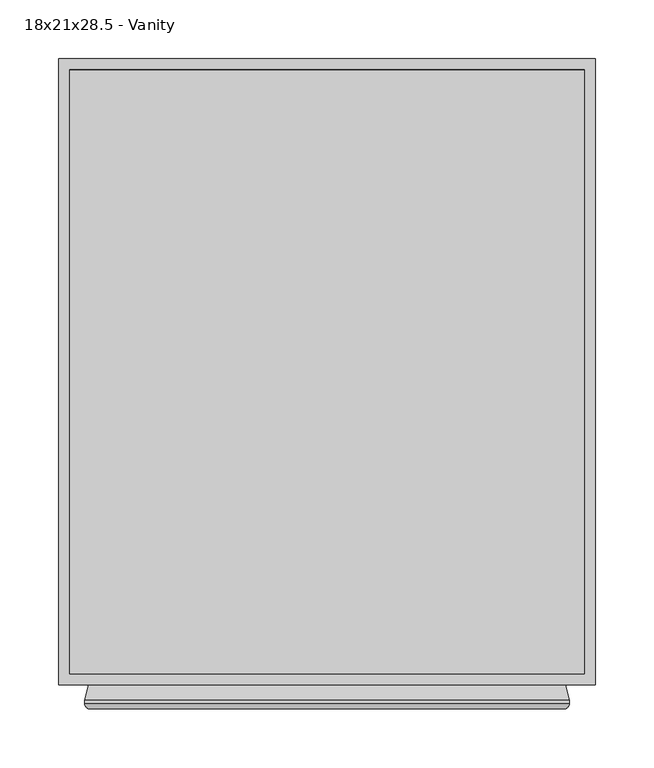
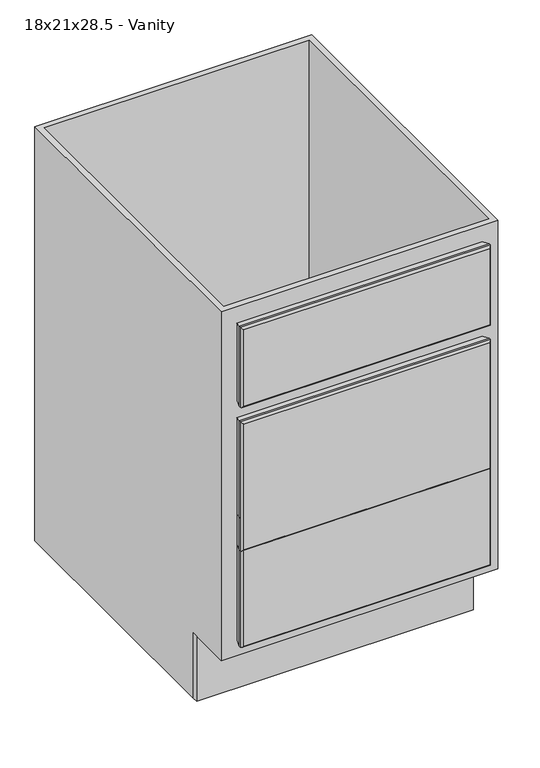
"""IFC4 building model written with IfcOpenShell, lengths in millimetres: furniture geometry, Cabinet-Base-Merillat-Three_Drawer-Marlin : 18x21x28.5 - Vanity."""

from ifc_helpers import new_model, si_unit, frame, origin, origin_with_axes, place, context, project, spatial, polyline, ellipse_curve, outline, extrude, faceted_brep, source, transform, mapped, element, save
from ifc_brep_helpers import plane_surface, cylinder_surface, advanced_brep


def furniture_18x21x28_5_vanity_0f894329(model_context):
    return source(origin(), model_context, "Body", "SolidModel", [
        advanced_brep(
        [(-184.5408026, -629.92, 530.3035075), (-184.5408026, -629.92, 311.0714925), (222.0162124, -629.92, 311.0714925), (222.0162124, -629.92, 530.3035075), (-184.1320951, -609.6, 311.4802), (-184.1320951, -609.6, 529.8948), (221.6075049, -609.6, 529.8948), (221.6075049, -609.6, 311.4802), (-187.6372951, -625.4496, 533.4), (-187.6372951, -622.681, 533.4), (-187.6372951, -622.681, 307.975), (-187.6372951, -625.4496, 307.975), (225.1127049, -622.681, 307.975), (225.1127049, -625.4496, 307.975), (225.1127049, -622.681, 533.4), (225.1127049, -625.4496, 533.4)],
        [
            (0, 1),
            (1, 2),
            (2, 3),
            (3, 0),
            (4, 5),
            (5, 6),
            (6, 7),
            (7, 4),
            (8, 9),
            (9, 10),
            (10, 11),
            (11, 8),
            (10, 12),
            (12, 13),
            (13, 11),
            (12, 14),
            (14, 15),
            (15, 13),
            (8, 15),
            (14, 9),
            (11, 1, ellipse_curve(frame((-182.8620951, -625.4496, 312.7502), z_axis=(-0.7071067811865475, 0.0, 0.7071067811865475), x_axis=(-0.7071067811865474, 0.0, -0.7071067811865476)), 6.7531526, 4.7752)),
            (0, 8, ellipse_curve(frame((-182.8620951, -625.4496, 528.6248), z_axis=(-0.7071067811865475, 0.0, -0.7071067811865475), x_axis=(0.7071067811865474, 0.0, -0.7071067811865476)), 6.7531526, 4.7752)),
            (4, 10),
            (9, 5),
            (13, 2, ellipse_curve(frame((220.3375049, -625.4496, 312.7502), z_axis=(-0.7071067811865475, 0.0, -0.7071067811865475), x_axis=(0.7071067811865476, 0.0, -0.7071067811865474)), 6.7531526, 4.7752)),
            (7, 12),
            (15, 3, ellipse_curve(frame((220.3375049, -625.4496, 528.6248), z_axis=(0.7071067811865475, 0.0, -0.7071067811865475), x_axis=(0.7071067811865474, 0.0, 0.7071067811865476)), 6.7531526, 4.7752)),
            (6, 14),
        ],
        [
            plane_surface(frame((-187.6372951, -629.92, 533.4), z_axis=(0.0, -1.0, 0.0), x_axis=(0.0, 0.0, -1.0))),
            plane_surface(frame((-187.6372951, -609.6, 533.4), z_axis=(0.0, 1.0, 0.0), x_axis=(0.0, 0.0, 1.0))),
            plane_surface(frame((-187.6372951, -629.92, 533.4), z_axis=(-1.0, 0.0, 0.0), x_axis=(0.0, 1.0, 0.0))),
            plane_surface(frame((-187.6372951, -629.92, 307.975), z_axis=(0.0, 0.0, -1.0), x_axis=(0.0, 1.0, 0.0))),
            plane_surface(frame((225.1127049, -629.92, 307.975), z_axis=(1.0, 0.0, 0.0), x_axis=(0.0, 1.0, 0.0))),
            plane_surface(frame((225.1127049, -629.92, 533.4), z_axis=(0.0, 0.0, 1.0), x_axis=(0.0, 1.0, 0.0))),
            cylinder_surface(frame((-182.8620951, -625.4496, 533.4), z_axis=(0.0, 0.0, -1.0), x_axis=(0.0, 1.0, 0.0)), 4.7752),
            plane_surface(frame((-187.6372951, -622.681, 533.4), z_axis=(-0.9659229350723619, 0.25882983502910506, 0.0), x_axis=(0.0, 0.0, -1.0))),
            cylinder_surface(frame((-187.6372951, -625.4496, 312.7502), z_axis=(1.0, 0.0, 0.0), x_axis=(0.0, 1.0, 0.0)), 4.7752),
            plane_surface(frame((-187.6372951, -622.681, 307.975), z_axis=(0.0, 0.25882983502910506, -0.9659229350723619), x_axis=(1.0, 0.0, 0.0))),
            cylinder_surface(frame((220.3375049, -625.4496, 307.975), z_axis=(0.0, 0.0, 1.0), x_axis=(0.0, 1.0, 0.0)), 4.7752),
            plane_surface(frame((225.1127049, -622.681, 307.975), z_axis=(0.9659229350723619, 0.25882983502910506, 0.0), x_axis=(0.0, 0.0, 1.0))),
            cylinder_surface(frame((225.1127049, -625.4496, 528.6248), z_axis=(-1.0, 0.0, 0.0), x_axis=(0.0, 1.0, 0.0)), 4.7752),
            plane_surface(frame((225.1127049, -622.681, 533.4), z_axis=(0.0, 0.25882983502910506, 0.9659229350723619), x_axis=(-1.0, 0.0, 0.0))),
        ],
        [
            (0, [[1, 2, 3, 4]]),
            (1, [[5, 6, 7, 8]]),
            (2, [[9, 10, 11, 12]]),
            (3, [[-11, 13, 14, 15]]),
            (4, [[-14, 16, 17, 18]]),
            (5, [[-9, 19, -17, 20]]),
            (6, [[21, -1, 22, -12]]),
            (7, [[23, -10, 24, -5]]),
            (8, [[-21, -15, 25, -2]]),
            (9, [[-23, -8, 26, -13]]),
            (10, [[-25, -18, 27, -3]]),
            (11, [[-26, -7, 28, -16]]),
            (12, [[-22, -4, -27, -19]]),
            (13, [[-24, -20, -28, -6]]),
        ],
    ),
        advanced_brep(
        [(-184.5408026, -629.92, 695.4035075), (-184.5408026, -629.92, 561.8964925), (222.0162124, -629.92, 561.8964925), (222.0162124, -629.92, 695.4035075), (-184.1320951, -609.6, 562.3052), (-184.1320951, -609.6, 694.9948), (221.6075049, -609.6, 694.9948), (221.6075049, -609.6, 562.3052), (-187.6372951, -625.4496, 698.5), (-187.6372951, -622.681, 698.5), (-187.6372951, -622.681, 558.8), (-187.6372951, -625.4496, 558.8), (225.1127049, -622.681, 558.8), (225.1127049, -625.4496, 558.8), (225.1127049, -622.681, 698.5), (225.1127049, -625.4496, 698.5)],
        [
            (0, 1),
            (1, 2),
            (2, 3),
            (3, 0),
            (4, 5),
            (5, 6),
            (6, 7),
            (7, 4),
            (8, 9),
            (9, 10),
            (10, 11),
            (11, 8),
            (10, 12),
            (12, 13),
            (13, 11),
            (12, 14),
            (14, 15),
            (15, 13),
            (8, 15),
            (14, 9),
            (11, 1, ellipse_curve(frame((-182.8620951, -625.4496, 563.5752), z_axis=(-0.7071067811865475, 0.0, 0.7071067811865475), x_axis=(-0.7071067811865474, 0.0, -0.7071067811865476)), 6.7531526, 4.7752)),
            (0, 8, ellipse_curve(frame((-182.8620951, -625.4496, 693.7248), z_axis=(-0.7071067811865475, 0.0, -0.7071067811865475), x_axis=(0.7071067811865474, 0.0, -0.7071067811865476)), 6.7531526, 4.7752)),
            (4, 10),
            (9, 5),
            (13, 2, ellipse_curve(frame((220.3375049, -625.4496, 563.5752), z_axis=(-0.7071067811865475, 0.0, -0.7071067811865475), x_axis=(0.7071067811865476, 0.0, -0.7071067811865474)), 6.7531526, 4.7752)),
            (7, 12),
            (15, 3, ellipse_curve(frame((220.3375049, -625.4496, 693.7248), z_axis=(0.7071067811865475, 0.0, -0.7071067811865475), x_axis=(0.7071067811865474, 0.0, 0.7071067811865476)), 6.7531526, 4.7752)),
            (6, 14),
        ],
        [
            plane_surface(frame((-187.6372951, -629.92, 698.5), z_axis=(0.0, -1.0, 0.0), x_axis=(0.0, 0.0, -1.0))),
            plane_surface(frame((-187.6372951, -609.6, 698.5), z_axis=(0.0, 1.0, 0.0), x_axis=(0.0, 0.0, 1.0))),
            plane_surface(frame((-187.6372951, -629.92, 698.5), z_axis=(-1.0, 0.0, 0.0), x_axis=(0.0, 1.0, 0.0))),
            plane_surface(frame((-187.6372951, -629.92, 558.8), z_axis=(0.0, 0.0, -1.0), x_axis=(0.0, 1.0, 0.0))),
            plane_surface(frame((225.1127049, -629.92, 558.8), z_axis=(1.0, 0.0, 0.0), x_axis=(0.0, 1.0, 0.0))),
            plane_surface(frame((225.1127049, -629.92, 698.5), z_axis=(0.0, 0.0, 1.0), x_axis=(0.0, 1.0, 0.0))),
            cylinder_surface(frame((-182.8620951, -625.4496, 698.5), z_axis=(0.0, 0.0, -1.0), x_axis=(0.0, 1.0, 0.0)), 4.7752),
            plane_surface(frame((-187.6372951, -622.681, 698.5), z_axis=(-0.9659229350723619, 0.25882983502910506, 0.0), x_axis=(0.0, 0.0, -1.0))),
            cylinder_surface(frame((-187.6372951, -625.4496, 563.5752), z_axis=(1.0, 0.0, 0.0), x_axis=(0.0, 1.0, 0.0)), 4.7752),
            plane_surface(frame((-187.6372951, -622.681, 558.8), z_axis=(0.0, 0.25882983502910506, -0.9659229350723619), x_axis=(1.0, 0.0, 0.0))),
            cylinder_surface(frame((220.3375049, -625.4496, 558.8), z_axis=(0.0, 0.0, 1.0), x_axis=(0.0, 1.0, 0.0)), 4.7752),
            plane_surface(frame((225.1127049, -622.681, 558.8), z_axis=(0.9659229350723619, 0.25882983502910506, 0.0), x_axis=(0.0, 0.0, 1.0))),
            cylinder_surface(frame((225.1127049, -625.4496, 693.7248), z_axis=(-1.0, 0.0, 0.0), x_axis=(0.0, 1.0, 0.0)), 4.7752),
            plane_surface(frame((225.1127049, -622.681, 698.5), z_axis=(0.0, 0.25882983502910506, 0.9659229350723619), x_axis=(-1.0, 0.0, 0.0))),
        ],
        [
            (0, [[1, 2, 3, 4]]),
            (1, [[5, 6, 7, 8]]),
            (2, [[9, 10, 11, 12]]),
            (3, [[-11, 13, 14, 15]]),
            (4, [[-14, 16, 17, 18]]),
            (5, [[-9, 19, -17, 20]]),
            (6, [[21, -1, 22, -12]]),
            (7, [[23, -10, 24, -5]]),
            (8, [[-21, -15, 25, -2]]),
            (9, [[-23, -8, 26, -13]]),
            (10, [[-25, -18, 27, -3]]),
            (11, [[-26, -7, 28, -16]]),
            (12, [[-22, -4, -27, -19]]),
            (13, [[-24, -20, -28, -6]]),
        ],
    ),
        advanced_brep(
        [(-184.5408026, -629.92, 362.0285075), (-184.5408026, -629.92, 142.7964925), (222.0162124, -629.92, 142.7964925), (222.0162124, -629.92, 362.0285075), (-184.1320951, -609.6, 143.2052), (-184.1320951, -609.6, 361.6198), (221.6075049, -609.6, 361.6198), (221.6075049, -609.6, 143.2052), (-187.6372951, -625.4496, 365.125), (-187.6372951, -622.681, 365.125), (-187.6372951, -622.681, 139.7), (-187.6372951, -625.4496, 139.7), (225.1127049, -622.681, 139.7), (225.1127049, -625.4496, 139.7), (225.1127049, -622.681, 365.125), (225.1127049, -625.4496, 365.125)],
        [
            (0, 1),
            (1, 2),
            (2, 3),
            (3, 0),
            (4, 5),
            (5, 6),
            (6, 7),
            (7, 4),
            (8, 9),
            (9, 10),
            (10, 11),
            (11, 8),
            (10, 12),
            (12, 13),
            (13, 11),
            (12, 14),
            (14, 15),
            (15, 13),
            (8, 15),
            (14, 9),
            (11, 1, ellipse_curve(frame((-182.8620951, -625.4496, 144.4752), z_axis=(-0.7071067811865475, 0.0, 0.7071067811865475), x_axis=(-0.7071067811865474, 0.0, -0.7071067811865476)), 6.7531526, 4.7752)),
            (0, 8, ellipse_curve(frame((-182.8620951, -625.4496, 360.3498), z_axis=(-0.7071067811865475, 0.0, -0.7071067811865475), x_axis=(0.7071067811865474, 0.0, -0.7071067811865476)), 6.7531526, 4.7752)),
            (4, 10),
            (9, 5),
            (13, 2, ellipse_curve(frame((220.3375049, -625.4496, 144.4752), z_axis=(-0.7071067811865475, 0.0, -0.7071067811865475), x_axis=(0.7071067811865476, 0.0, -0.7071067811865474)), 6.7531526, 4.7752)),
            (7, 12),
            (15, 3, ellipse_curve(frame((220.3375049, -625.4496, 360.3498), z_axis=(0.7071067811865475, 0.0, -0.7071067811865475), x_axis=(0.7071067811865474, 0.0, 0.7071067811865476)), 6.7531526, 4.7752)),
            (6, 14),
        ],
        [
            plane_surface(frame((-187.6372951, -629.92, 365.125), z_axis=(0.0, -1.0, 0.0), x_axis=(0.0, 0.0, -1.0))),
            plane_surface(frame((-187.6372951, -609.6, 365.125), z_axis=(0.0, 1.0, 0.0), x_axis=(0.0, 0.0, 1.0))),
            plane_surface(frame((-187.6372951, -629.92, 365.125), z_axis=(-1.0, 0.0, 0.0), x_axis=(0.0, 1.0, 0.0))),
            plane_surface(frame((-187.6372951, -629.92, 139.7), z_axis=(0.0, 0.0, -1.0), x_axis=(0.0, 1.0, 0.0))),
            plane_surface(frame((225.1127049, -629.92, 139.7), z_axis=(1.0, 0.0, 0.0), x_axis=(0.0, 1.0, 0.0))),
            plane_surface(frame((225.1127049, -629.92, 365.125), z_axis=(0.0, 0.0, 1.0), x_axis=(0.0, 1.0, 0.0))),
            cylinder_surface(frame((-182.8620951, -625.4496, 365.125), z_axis=(0.0, 0.0, -1.0), x_axis=(0.0, 1.0, 0.0)), 4.7752),
            plane_surface(frame((-187.6372951, -622.681, 365.125), z_axis=(-0.9659229350723619, 0.25882983502910506, 0.0), x_axis=(0.0, 0.0, -1.0))),
            cylinder_surface(frame((-187.6372951, -625.4496, 144.4752), z_axis=(1.0, 0.0, 0.0), x_axis=(0.0, 1.0, 0.0)), 4.7752),
            plane_surface(frame((-187.6372951, -622.681, 139.7), z_axis=(0.0, 0.25882983502910506, -0.9659229350723619), x_axis=(1.0, 0.0, 0.0))),
            cylinder_surface(frame((220.3375049, -625.4496, 139.7), z_axis=(0.0, 0.0, 1.0), x_axis=(0.0, 1.0, 0.0)), 4.7752),
            plane_surface(frame((225.1127049, -622.681, 139.7), z_axis=(0.9659229350723619, 0.25882983502910506, 0.0), x_axis=(0.0, 0.0, 1.0))),
            cylinder_surface(frame((225.1127049, -625.4496, 360.3498), z_axis=(-1.0, 0.0, 0.0), x_axis=(0.0, 1.0, 0.0)), 4.7752),
            plane_surface(frame((225.1127049, -622.681, 365.125), z_axis=(0.0, 0.25882983502910506, 0.9659229350723619), x_axis=(-1.0, 0.0, 0.0))),
        ],
        [
            (0, [[1, 2, 3, 4]]),
            (1, [[5, 6, 7, 8]]),
            (2, [[9, 10, 11, 12]]),
            (3, [[-11, 13, 14, 15]]),
            (4, [[-14, 16, 17, 18]]),
            (5, [[-9, 19, -17, 20]]),
            (6, [[21, -1, 22, -12]]),
            (7, [[23, -10, 24, -5]]),
            (8, [[-21, -15, 25, -2]]),
            (9, [[-23, -8, 26, -13]]),
            (10, [[-25, -18, 27, -3]]),
            (11, [[-26, -7, 28, -16]]),
            (12, [[-22, -4, -27, -19]]),
            (13, [[-24, -20, -28, -6]]),
        ],
    ),
        extrude(outline(polyline([(-209.8622951, -538.95625), (-209.8622951, -529.43125), (247.3377049, -529.43125), (247.3377049, -538.95625), (-209.8622951, -538.95625)])), origin_with_axes(), (0.0, 0.0, 1.0), 114.3),
        faceted_brep([(247.3377049, -76.2, 0.0), (247.3377049, -529.43125, 0.0), (237.8127049, -529.43125, 0.0), (237.8127049, -85.725, 0.0), (-200.3372951, -85.725, 0.0), (-200.3372951, -529.43125, 0.0), (-209.8622951, -529.43125, 0.0), (-209.8622951, -76.2, 0.0), (-209.8622951, -76.2, 723.9), (247.3377049, -76.2, 723.9), (-209.8622951, -529.43125, 114.3), (-209.8622951, -609.6, 114.3), (-209.8622951, -609.6, 723.9), (247.3377049, -609.6, 723.9), (247.3377049, -609.6, 114.3), (247.3377049, -529.43125, 114.3), (237.8127049, -529.43125, 114.3), (237.8127049, -85.725, 114.3), (237.8127049, -600.075, 723.9), (237.8127049, -85.725, 723.9), (237.8127049, -85.725, 123.825), (237.8127049, -600.075, 123.825), (-200.3372951, -85.725, 114.3), (-200.3372951, -529.43125, 114.3), (-200.3372951, -85.725, 723.9), (-200.3372951, -600.075, 723.9), (-200.3372951, -600.075, 123.825), (-200.3372951, -85.725, 123.825)], [[[0, 1, 2, 3, 4, 5, 6, 7]], [[0, 7, 8, 9]], [[7, 6, 10, 11, 12, 8]], [[1, 0, 9, 13, 14, 15]], [[3, 2, 16, 17]], [[18, 19, 20, 21]], [[5, 4, 22, 23]], [[24, 25, 26, 27]], [[4, 3, 17, 22]], [[19, 24, 27, 20]], [[9, 8, 12, 13], [19, 18, 25, 24]], [[14, 11, 10, 23, 22, 17, 16, 15]], [[13, 12, 11, 14]], [[25, 18, 21, 26]], [[21, 20, 27, 26]], [[6, 5, 23, 10]], [[2, 1, 15, 16]]]),
    ])


if __name__ == "__main__":
    model = new_model("IFC4")
    model_context = context("Model", 3, world=origin())
    ifc_project = project(units=[si_unit("LENGTHUNIT", "METRE", prefix="MILLI")], contexts=[model_context])
    site = spatial("IfcSite", under=ifc_project)
    building = spatial("IfcBuilding", under=site)
    placement = place(None, origin())
    furniture_18x21x28_5_vanity_shape = furniture_18x21x28_5_vanity_0f894329(model_context)
    element("IfcFurniture", 1, ObjectType="Cabinet-Base-Merillat-Three_Drawer-Marlin : 18x21x28.5 - Vanity", at=placement, inside=building, context=model_context, shape_type="MappedRepresentation", body=[
        mapped(furniture_18x21x28_5_vanity_shape, transform((0.0, 0.0, 0.0), x_axis=(1.0, 0.0, 0.0), y_axis=(0.0, 1.0, 0.0), z_axis=(0.0, 0.0, 1.0))),
    ])
    save(model, "model.ifc")

# Revit data of these elements
# Type "Cabinet-Base-Merillat-Three_Drawer-Marlin : 18x21x28.5 - Vanity"
#   URL = "http://www.merillat.com"
#   Toe Kick Note = "Toe Kick Covering is not included. To be purchased Separately."
#   Product Page URL = "http://www.merillat.com//our-products/rooms/bathroom/"
#   Product Line = "Express"
#   Product Group = "Vanity Cabinet"
#   Product Documentation Link = "http://merillatbusiness.com/customer-resources/product-line-resources/merillat-classic/"
#   Model = "VD18-3D"
#   Manufacturer = "Merillat"
#   Finish = "Wood"
#   Description = "Vanity Drawer Three Drawer"
#   Construction Type = "Base Three Drawer"
#   Cabinet Construction Note = "One standard height top drawer and two deep drawers below"
#   Assembly Code = "C1030410"
#   Top and Bottom Spacing = 0' - 1"
#   Toe Kick Height = 0' - 4 1/2"
#   Toe Kick Depth = 0' - 2 25/32"
#   Standard Drawer Height = 0' - 5 1/2"
#   Depth = 1' - 9"
#   Height = 2' - 4 1/2"
#   Width = 1' - 6"
#   Deep Drawer Height = 0' - 8 7/8"
#   Cabinet Shell = 0' - 0 3/8"
#   Cabinet Door Width = 1' - 4 1/4"
#   COBie.Type = no
#   Partial Overlay = yes
#   Full Overlay = no
#   Toe Kick Material = Wood - Merillat - Raw Particle Board
#   Door Drawer Material = Wood - Merillat - Pecan(1)
#   Cabinet Material = Wood - Merillat - Pecan(1)
#   Cabinet Drawer Style = element 795666
# Element 1 (IfcFurniture, "Cabinet-Base-Merillat-Three_Drawer-Marlin : 18x21x28.5 - Vanity")
#   Materials on its faces: "Wood - Merillat - Pecan(1)", "Wood - Merillat - Raw Particle Board"
# Materials
#   "Wood - Merillat - Raw Particle Board": class "Plastic", colour RGB 80 80 80, transparency 0, Description = "Plastic Laminate - Navy", Cost = 0
#   "Wood - Merillat - Pecan(1)": class "Wood", colour RGB 108 67 43, transparency 0, Cost = 0
